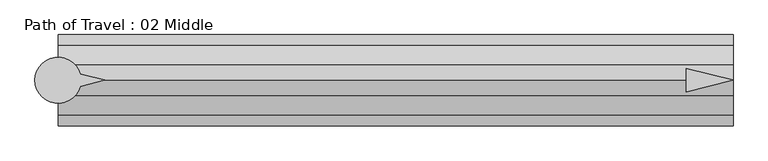
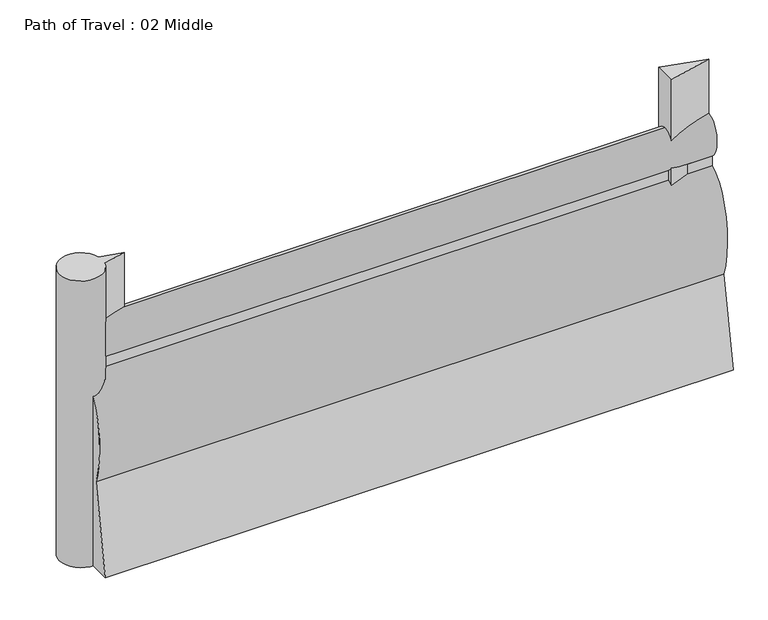
"""IFC4 building model written with IfcOpenShell, lengths in millimetres: proxy geometry, Path of Travel : 02 Middle."""

import ifcopenshell
import ifcopenshell.guid

model = None  # the IFC model being written
_history = None  # IfcOwnerHistory: only IFC2X3 demands one
_inside = {}  # id of a spatial element -> (the spatial element, [elements in it])
_under = {}  # id of a project, library or spatial element -> (it, [spatial elements below it])
_declared = {}  # id of a project -> (the project, [libraries it declares])
_typed = {}  # id of a type object -> (the type object, [elements of that type])
_made_of = {}  # id of a material, layer set ... -> (it, [elements and type objects made of it])


def new_model(schema):
    """Start an empty IFC model of exactly this schema.

    Asked for "IFC4X3", IfcOpenShell would pick the latest addendum, in which some entities
    have other attributes; the version numbers below select the first issue.
    IFC2X3 requires an IfcOwnerHistory on every rooted entity: one is made here for all.
    """
    global model, _history
    if schema == "IFC4X3":
        model = ifcopenshell.file(schema_version=(4, 3, 0, 0))
    else:
        model = ifcopenshell.file(schema=schema)
    _inside.clear()
    _under.clear()
    _declared.clear()
    _typed.clear()
    _made_of.clear()
    _history = None
    if model.schema == "IFC2X3":
        org = make("IfcOrganization", Name="unknown")
        user = make(
            "IfcPersonAndOrganization",
            ThePerson=make("IfcPerson", FamilyName="unknown"),
            TheOrganization=org,
        )
        app = make(
            "IfcApplication",
            ApplicationDeveloper=org,
            Version="unknown",
            ApplicationFullName="unknown",
            ApplicationIdentifier="unknown",
        )
        _history = make(
            "IfcOwnerHistory",
            OwningUser=user,
            OwningApplication=app,
            ChangeAction="ADDED",
            CreationDate=0,
        )
    return model


def make(cls, **values):
    """One entity of the class cls with the attributes given. An attribute that is None is left unset."""
    return model.create_entity(
        cls, **{name: value for name, value in values.items() if value is not None}
    )


def rooted(cls, **values):
    """An entity with a GlobalId (a new one), such as an element, a storey or a relation."""
    return make(cls, GlobalId=ifcopenshell.guid.new(), OwnerHistory=_history, **values)


def si_unit(unit_type, name, prefix=None):
    """IfcSIUnit, for example si_unit("LENGTHUNIT", "METRE", prefix="MILLI")."""
    return make("IfcSIUnit", UnitType=unit_type, Prefix=prefix, Name=name)


def assignment(units):
    """IfcUnitAssignment: the units of a project."""
    return None if units is None else make("IfcUnitAssignment", Units=units)


def point(xyz):
    """IfcCartesianPoint."""
    return None if xyz is None else make("IfcCartesianPoint", Coordinates=xyz)


def direction(xyz):
    """IfcDirection."""
    return None if xyz is None else make("IfcDirection", DirectionRatios=xyz)


def frame(location, z_axis=None, x_axis=None):
    """IfcAxis2Placement3D, a coordinate frame: its origin and axes. An axis left out is left unset."""
    return make(
        "IfcAxis2Placement3D",
        Location=point(location),
        Axis=direction(z_axis),
        RefDirection=direction(x_axis),
    )


def frame_2d(location, x_axis=None):
    """IfcAxis2Placement2D, a coordinate frame in the plane: its origin and x axis."""
    return make(
        "IfcAxis2Placement2D", Location=point(location), RefDirection=direction(x_axis)
    )


def origin():
    """The frame at (0, 0, 0) with its axes left unset."""
    return frame((0.0, 0.0, 0.0))


def origin_with_axes():
    """The frame at (0, 0, 0) with the z axis (0, 0, 1) and the x axis (1, 0, 0) written out."""
    return frame((0.0, 0.0, 0.0), z_axis=(0.0, 0.0, 1.0), x_axis=(1.0, 0.0, 0.0))


def place(relative_to, where):
    """IfcLocalPlacement: puts the frame where relative to a parent placement (None: the world)."""
    return make(
        "IfcLocalPlacement", PlacementRelTo=relative_to, RelativePlacement=where
    )


def context(
    kind, dimensions, precision=None, world=None, true_north=None, identifier=None
):
    """IfcGeometricRepresentationContext, for example the 3D "Model" context."""
    return make(
        "IfcGeometricRepresentationContext",
        ContextIdentifier=identifier,
        ContextType=kind,
        CoordinateSpaceDimension=dimensions,
        Precision=precision,
        WorldCoordinateSystem=world,
        TrueNorth=true_north,
    )


def project(units=None, contexts=None):
    """IfcProject with its units and contexts."""
    return rooted(
        "IfcProject",
        Name="project",
        RepresentationContexts=contexts,
        UnitsInContext=assignment(units),
    )


def spatial(cls, under=None, at=None, **own):
    """A site, building, storey or space (cls), placed at a placement, below another one or the project."""
    s = rooted(cls, ObjectPlacement=at, **own)
    if under is not None:
        _under.setdefault(under.id(), (under, []))[1].append(s)
    return s


def polyline(points):
    """IfcPolyline through the points."""
    return make("IfcPolyline", Points=[point(p) for p in points])


def circle_curve(where, radius):
    """IfcCircle in the frame where."""
    return make("IfcCircle", Position=where, Radius=radius)


def ellipse_curve(where, semi_axis1, semi_axis2):
    """IfcEllipse in the frame where."""
    return make(
        "IfcEllipse", Position=where, SemiAxis1=semi_axis1, SemiAxis2=semi_axis2
    )


def trimmed(basis, trim1, trim2, sense, master):
    """IfcTrimmedCurve: the piece of a basis curve between two trims."""
    return make(
        "IfcTrimmedCurve",
        BasisCurve=basis,
        Trim1=trim1,
        Trim2=trim2,
        SenseAgreement=sense,
        MasterRepresentation=master,
    )


def segment(curve, same_sense, transition):
    """IfcCompositeCurveSegment."""
    return make(
        "IfcCompositeCurveSegment",
        Transition=transition,
        SameSense=same_sense,
        ParentCurve=curve,
    )


def composite_curve(segments, self_intersect=None):
    """IfcCompositeCurve: segments joined end to end."""
    return make("IfcCompositeCurve", Segments=segments, SelfIntersect=self_intersect)


def outline(outer, holes=None, kind="AREA"):
    """IfcArbitraryClosedProfileDef: a profile drawn as a closed curve; with holes, ...WithVoids."""
    if holes is None:
        return make("IfcArbitraryClosedProfileDef", ProfileType=kind, OuterCurve=outer)
    return make(
        "IfcArbitraryProfileDefWithVoids",
        ProfileType=kind,
        OuterCurve=outer,
        InnerCurves=holes,
    )


def extrude(swept, where, along, depth):
    """IfcExtrudedAreaSolid: the profile swept, set in the frame where, extruded along a direction by depth."""
    return make(
        "IfcExtrudedAreaSolid",
        SweptArea=swept,
        Position=where,
        ExtrudedDirection=direction(along),
        Depth=depth,
    )


def shape(context_of_items, identifier, shape_type, items):
    """IfcShapeRepresentation: the items that make up one representation, for example the "Body"."""
    return make(
        "IfcShapeRepresentation",
        ContextOfItems=context_of_items,
        RepresentationIdentifier=identifier,
        RepresentationType=shape_type,
        Items=items,
    )


def source(mapping_origin, context_of_items, identifier, shape_type, items):
    """IfcRepresentationMap: a shape defined once, which mapped items show again and again."""
    return make(
        "IfcRepresentationMap",
        MappingOrigin=mapping_origin,
        MappedRepresentation=shape(context_of_items, identifier, shape_type, items),
    )


def transform(
    local_origin,
    x_axis=None,
    y_axis=None,
    z_axis=None,
    scale=None,
    scale2=None,
    scale3=None,
    uniform=True,
):
    """IfcCartesianTransformationOperator3D, or its non-uniform kind. x_axis, y_axis, z_axis: its Axis1, 2, 3."""
    if uniform:
        return make(
            "IfcCartesianTransformationOperator3D",
            Axis1=direction(x_axis),
            Axis2=direction(y_axis),
            LocalOrigin=point(local_origin),
            Scale=scale,
            Axis3=direction(z_axis),
        )
    return make(
        "IfcCartesianTransformationOperator3DnonUniform",
        Axis1=direction(x_axis),
        Axis2=direction(y_axis),
        LocalOrigin=point(local_origin),
        Scale=scale,
        Axis3=direction(z_axis),
        Scale2=scale2,
        Scale3=scale3,
    )


def mapped(mapping_source, mapping_target):
    """IfcMappedItem: shows the shape of a source again, moved by a transform."""
    return make(
        "IfcMappedItem", MappingSource=mapping_source, MappingTarget=mapping_target
    )


def made_of(thing, what):
    """Note that an element or type object is made of a material, layer set ...; save() writes the relation."""
    if what is not None:
        _made_of.setdefault(what.id(), (what, []))[1].append(thing)
    return thing


def element(
    cls,
    number,
    at=None,
    inside=None,
    cuts=None,
    type_object=None,
    material=None,
    context=None,
    identifier="Body",
    shape_type=None,
    held_by="IfcProductDefinitionShape",
    body=None,
    shapes=None,
    **own,
):
    """One element of the class cls, such as IfcWall. Its Tag is "e" and its number.

    at: its placement. inside: the storey or other place that contains it. cuts: it is an
    opening in that element (IfcRelVoidsElement). A single representation is given by context,
    identifier, shape_type and body (its items); several are given by shapes. held_by: the class
    of the entity that holds the representations. save() writes the other relations.
    """
    e = rooted(cls, Tag="e%d" % number, ObjectPlacement=at, **own)
    if body is not None:
        shapes = [shape(context, identifier, shape_type, body)]
    if shapes is not None:
        e.Representation = make(held_by, Representations=shapes)
    if inside is not None:
        _inside.setdefault(inside.id(), (inside, []))[1].append(e)
    if cuts is not None:
        rooted(
            "IfcRelVoidsElement", RelatingBuildingElement=cuts, RelatedOpeningElement=e
        )
    if type_object is not None:
        _typed.setdefault(type_object.id(), (type_object, []))[1].append(e)
    return made_of(e, material)


def aggregate(whole, parts):
    """IfcRelAggregates: a whole, such as a stair, and the parts it consists of."""
    return rooted("IfcRelAggregates", RelatingObject=whole, RelatedObjects=parts)


def save(model, path):
    """Write the relations noted so far, then the file.

    IfcRelAggregates (storeys below a building ...), IfcRelContainedInSpatialStructure (elements
    in a storey), IfcRelDefinesByType, IfcRelAssociatesMaterial and IfcRelDeclares: one each for
    every whole, place, type object, material and project.
    """
    for whole, parts in _under.values():
        aggregate(whole, parts)
    for where, things in _inside.values():
        rooted(
            "IfcRelContainedInSpatialStructure",
            RelatedElements=things,
            RelatingStructure=where,
        )
    for kind, things in _typed.values():
        rooted("IfcRelDefinesByType", RelatedObjects=things, RelatingType=kind)
    for what, things in _made_of.values():
        rooted("IfcRelAssociatesMaterial", RelatedObjects=things, RelatingMaterial=what)
    for by, libraries in _declared.values():
        rooted("IfcRelDeclares", RelatingContext=by, RelatedDefinitions=libraries)
    model.write(path)


def plane_surface(at):
    """IfcPlane: the flat surface through the origin of the frame at, square to its z axis."""
    return make("IfcPlane", Position=at)


def extruded_surface(curve, direction_of_extrusion, depth):
    """IfcSurfaceOfLinearExtrusion: the curve pushed along a direction by depth."""
    return make(
        "IfcSurfaceOfLinearExtrusion",
        SweptCurve=make("IfcArbitraryOpenProfileDef", ProfileType="CURVE", Curve=curve),
        ExtrudedDirection=direction(direction_of_extrusion),
        Depth=depth,
    )


def advanced_brep(points, edges, surfaces, faces):
    """IfcAdvancedBrep: a solid bounded by faces that lie on surfaces and meet in shared edges.

    An edge is (start, end): straight between two places in points (the first is 0);
    or (start, end, curve); or (start, end, curve, False) where it runs against its curve.
    A face is (place in surfaces, loops), or (place, loops, False) where it looks against
    its surface's normal. A loop lists edges by number (the first is 1), with a minus sign
    where the edge is run from its end to its start. The first loop is the outer one.
    """
    corners = [point(p) for p in points]
    vertices = [make("IfcVertexPoint", VertexGeometry=c) for c in corners]
    made = []
    for start, end, *more in edges:
        made.append(
            make(
                "IfcEdgeCurve",
                EdgeStart=vertices[start],
                EdgeEnd=vertices[end],
                EdgeGeometry=more[0] if more else make("IfcPolyline", Points=[corners[start], corners[end]]),
                SameSense=more[1] if len(more) > 1 else True,
            )
        )
    hull = []
    for where, loops, *sense in faces:
        bounds = []
        for j, loop in enumerate(loops):
            ring = [make("IfcOrientedEdge", EdgeElement=made[abs(k) - 1], Orientation=k > 0) for k in loop]
            bounds.append(
                make(
                    "IfcFaceOuterBound" if j == 0 else "IfcFaceBound",
                    Bound=make("IfcEdgeLoop", EdgeList=ring),
                    Orientation=True,
                )
            )
        hull.append(make("IfcAdvancedFace", Bounds=bounds, FaceSurface=surfaces[where], SameSense=sense[0] if sense else True))
    return make("IfcAdvancedBrep", Outer=make("IfcClosedShell", CfsFaces=hull))


def path_of_travel_02_middle_5bade7f2(model_context):
    return source(origin(), model_context, "Body", "SolidModel", [
        advanced_brep(
        [(227.5554837, 0.0, 1727.2), (227.5554837, 42.9018657, 1436.6534209), (227.5554837, 42.9018657, 1363.4763406), (227.5554837, 184.1186263, 643.4144547), (227.5554837, 297.5699544, 0.0), (227.5554837, 145.6574193, 0.0), (227.5554837, 0.0, 584.2), (227.5554837, -145.6574193, 0.0), (227.5554837, -297.5699544, 0.0), (227.5554837, -184.1186263, 643.4144547), (227.5554837, -42.9018657, 1363.4763406), (227.5554837, -42.9018657, 1436.6534209), (4635.9128813, 0.0, 1727.2), (4635.9128813, -42.9018657, 1436.6534209), (4635.9128813, -42.9018657, 1363.4763406), (4635.9128813, -184.1186263, 643.4144547), (4635.9128813, -297.5699544, 0.0), (4635.9128813, -145.6574193, 0.0), (4635.9128813, 0.0, 584.2), (4635.9128813, 145.6574193, 0.0), (4635.9128813, 297.5699544, 0.0), (4635.9128813, 184.1186263, 643.4144547), (4635.9128813, 42.9018657, 1363.4763406), (4635.9128813, 42.9018657, 1436.6534209)],
        [
            (0, 1, ellipse_curve(frame((227.5554837, 0.0, 1574.8), z_axis=(-1.0, 0.0, 0.0), x_axis=(0.0, 0.0, 1.0)), 152.4, 101.6)),
            (1, 2),
            (2, 3, ellipse_curve(frame((227.5554837, 0.0, 914.4), z_axis=(-1.0, 0.0, 0.0), x_axis=(0.0, 0.0, -1.0)), 457.2, 228.6)),
            (3, 4),
            (4, 5),
            (5, 6),
            (6, 7),
            (7, 8),
            (8, 9),
            (9, 10, ellipse_curve(frame((227.5554837, 0.0, 914.4), z_axis=(-1.0, 0.0, 0.0), x_axis=(0.0, 0.0, -1.0)), 457.2, 228.6)),
            (10, 11),
            (11, 0, ellipse_curve(frame((227.5554837, 0.0, 1574.8), z_axis=(-1.0, 0.0, 0.0), x_axis=(0.0, 0.0, 1.0)), 152.4, 101.6)),
            (12, 13, ellipse_curve(frame((4635.9128813, 0.0, 1574.8), z_axis=(1.0, 0.0, 0.0), x_axis=(0.0, 0.0, 1.0)), 152.4, 101.6)),
            (13, 14),
            (14, 15, ellipse_curve(frame((4635.9128813, 0.0, 914.4), z_axis=(1.0, 0.0, 0.0), x_axis=(0.0, 0.0, -1.0)), 457.2, 228.6)),
            (15, 16),
            (16, 17),
            (17, 18),
            (18, 19),
            (19, 20),
            (20, 21),
            (21, 22, ellipse_curve(frame((4635.9128813, 0.0, 914.4), z_axis=(1.0, 0.0, 0.0), x_axis=(0.0, 0.0, -1.0)), 457.2, 228.6)),
            (22, 23),
            (23, 12, ellipse_curve(frame((4635.9128813, 0.0, 1574.8), z_axis=(1.0, 0.0, 0.0), x_axis=(0.0, 0.0, 1.0)), 152.4, 101.6)),
            (0, 12),
            (23, 1),
            (22, 2),
            (21, 3),
            (20, 4),
            (19, 5),
            (18, 6),
            (17, 7),
            (16, 8),
            (15, 9),
            (14, 10),
            (13, 11),
        ],
        [
            plane_surface(frame((227.5554837, 0.0, 0.0), z_axis=(-1.0, 0.0, 0.0), x_axis=(0.0, 0.0, 1.0))),
            plane_surface(frame((4635.9128813, 0.0, 0.0), z_axis=(1.0, 0.0, 0.0), x_axis=(0.0, 0.0, 1.0))),
            extruded_surface(trimmed(ellipse_curve(frame((4635.9128813, 0.0, 1574.8), z_axis=(-1.0, 0.0, 0.0), x_axis=(0.0, 0.0, 1.0)), 152.4, 101.6), [point((4635.9128813, 0.0, 1727.2))], [point((4635.9128813, 42.9018657, 1436.6534209))], True, "CARTESIAN"), (-4408.3573976, 0.0, 0.0), 4408.3573976),
            plane_surface(frame((227.5554837, 42.9018657, 1436.6534209), z_axis=(0.0, 1.0, 0.0), x_axis=(1.0, 0.0, 0.0))),
            extruded_surface(trimmed(ellipse_curve(frame((4635.9128813, 0.0, 914.4), z_axis=(-1.0, 0.0, 0.0), x_axis=(0.0, 0.0, -1.0)), 457.2, 228.6), [point((4635.9128813, 42.9018657, 1363.4763406))], [point((4635.9128813, 184.1186263, 643.4144547))], True, "CARTESIAN"), (-4408.3573976, 0.0, 0.0), 4408.3573976),
            plane_surface(frame((227.5554837, 184.1186263, 643.4144547), z_axis=(0.0, 0.9848077530122078, 0.1736481776669322), x_axis=(1.0, 0.0, 0.0))),
            plane_surface(frame((227.5554837, 297.5699544, 0.0), z_axis=(0.0, 0.0, -1.0), x_axis=(1.0, 0.0, 0.0))),
            plane_surface(frame((227.5554837, 145.6574193, 0.0), z_axis=(0.0, -0.9702957262760199, -0.2419218955995739), x_axis=(1.0, 0.0, 0.0))),
            plane_surface(frame((227.5554837, 0.0, 584.2), z_axis=(0.0, 0.9702957262759961, -0.24192189559966923), x_axis=(1.0, 0.0, 0.0))),
            plane_surface(frame((227.5554837, -145.6574193, 0.0), z_axis=(0.0, 0.0, -1.0), x_axis=(1.0, 0.0, 0.0))),
            plane_surface(frame((227.5554837, -297.5699544, 0.0), z_axis=(0.0, -0.984807753012208, 0.17364817766693066), x_axis=(1.0, 0.0, 0.0))),
            extruded_surface(trimmed(ellipse_curve(frame((4635.9128813, 0.0, 914.4), z_axis=(-1.0, 0.0, 0.0), x_axis=(0.0, 0.0, -1.0)), 457.2, 228.6), [point((4635.9128813, -184.1186263, 643.4144547))], [point((4635.9128813, -42.9018657, 1363.4763406))], True, "CARTESIAN"), (-4408.3573976, 0.0, 0.0), 4408.3573976),
            plane_surface(frame((227.5554837, -42.9018657, 1363.4763406), z_axis=(0.0, -1.0, 0.0), x_axis=(1.0, 0.0, 0.0))),
            extruded_surface(trimmed(ellipse_curve(frame((4635.9128813, 0.0, 1574.8), z_axis=(-1.0, 0.0, 0.0), x_axis=(0.0, 0.0, 1.0)), 152.4, 101.6), [point((4635.9128813, -42.9018657, 1436.6534209))], [point((4635.9128813, 0.0, 1727.2))], True, "CARTESIAN"), (-4408.3573976, 0.0, 0.0), 4408.3573976),
        ],
        [
            (0, [[1, 2, 3, 4, 5, 6, 7, 8, 9, 10, 11, 12]]),
            (1, [[13, 14, 15, 16, 17, 18, 19, 20, 21, 22, 23, 24]]),
            (2, [[-1, 25, -24, 26]]),
            (3, [[-2, -26, -23, 27]]),
            (4, [[-3, -27, -22, 28]]),
            (5, [[-4, -28, -21, 29]]),
            (6, [[-5, -29, -20, 30]]),
            (7, [[-6, -30, -19, 31]]),
            (8, [[-7, -31, -18, 32]]),
            (9, [[-8, -32, -17, 33]]),
            (10, [[-9, -33, -16, 34]]),
            (11, [[-10, -34, -15, 35]]),
            (12, [[-11, -35, -14, 36]]),
            (13, [[-12, -36, -13, -25]]),
        ],
    ),
        extrude(outline(polyline([(4329.9077347, 76.2006338), (4635.9128813, 0.0), (4329.9077347, -76.2006338), (4329.9077347, 76.2006338)])), origin_with_axes(), (0.0, 0.0, 1.0), 2129.5973753),
        extrude(outline(composite_curve([segment(polyline([(372.7837828, 39.4440225), (531.182385, 0.0), (372.7837828, -39.4440225)]), True, "CONTINUOUS"), segment(trimmed(circle_curve(frame_2d((227.2200886, 0.0)), 150.8131956), [point((372.7837828, -39.4440225))], [point((372.7837828, 39.4440225))], False, "CARTESIAN"), True, "CONTINUOUS")], self_intersect=False)), origin_with_axes(), (0.0, 0.0, 1.0), 2129.5973753),
    ])


if __name__ == "__main__":
    model = new_model("IFC4")
    model_context = context("Model", 3, world=origin())
    ifc_project = project(units=[si_unit("LENGTHUNIT", "METRE", prefix="MILLI")], contexts=[model_context])
    site = spatial("IfcSite", under=ifc_project)
    building = spatial("IfcBuilding", under=site)
    placement = place(None, origin())
    path_of_travel_02_middle_shape = path_of_travel_02_middle_5bade7f2(model_context)
    element("IfcBuildingElementProxy", 1, Name="Path of Travel : 02 Middle", ObjectType="Path of Travel : 02 Middle", at=placement, inside=building, context=model_context, shape_type="MappedRepresentation", body=[
        mapped(path_of_travel_02_middle_shape, transform((0.0, 0.0, 0.0), x_axis=(1.0, 0.0, 0.0), y_axis=(0.0, 1.0, 0.0), z_axis=(0.0, 0.0, 1.0))),
    ])
    save(model, "model.ifc")

# Revit data of these elements
# Type "Path of Travel : 02 Middle"
#   Path of Egress [instance default] = 4' - 0"
#   built-in parameter 1001306 [instance default] = 4 (stored number, unit not read)
#   Dot at Start = no
#   Arrow in Middle = yes
#   Arrow at End = no
#   Egress Path = none
# Element 1 (IfcBuildingElementProxy, "Path of Travel : 02 Middle")
#   Path of Egress = 14' - 5.55738"
#   built-in parameter 1001306 = 14.4631 (stored number, unit not read)
#   Materials on its faces: "Egress Path Solid", "solid"
# Materials
#   "Egress Path Solid": class "Unassigned", colour RGB 255 128 64, transparency 0.75, Comments = "Rendering appearance not upgraded "
#   "solid": class "Generic", colour RGB 120 120 120, transparency 0, Cost = 0
